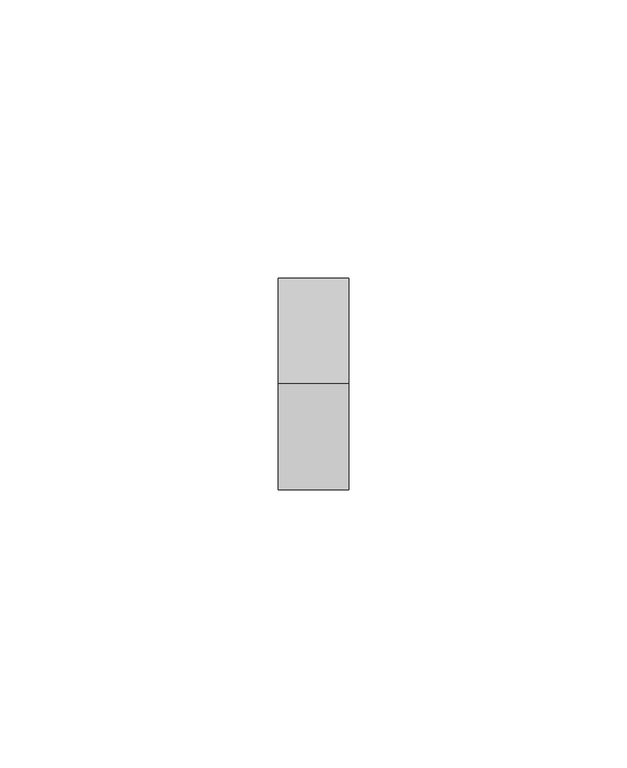
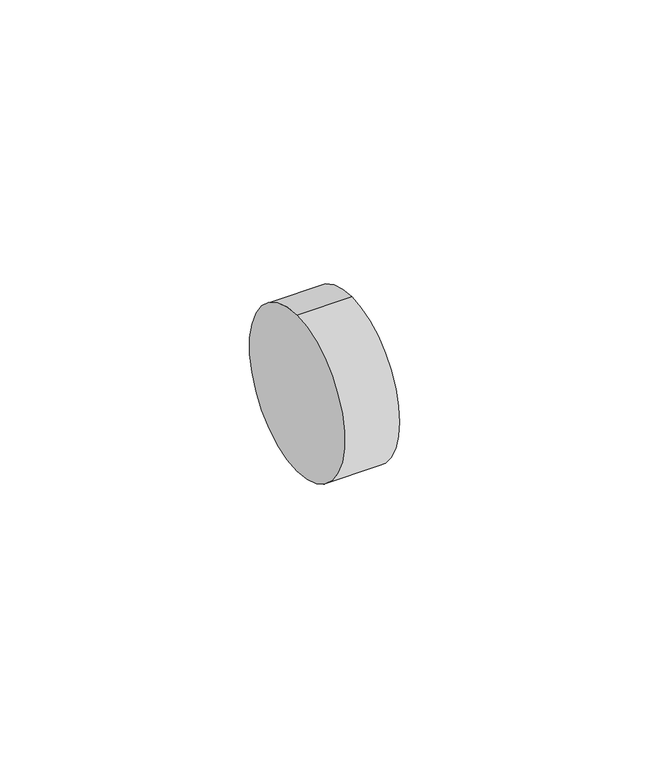
"""IFC4 building model written with IfcOpenShell, lengths in millimetres: proxy geometry, Bolt29:Bolt002:304741 : Bolt29:Bolt002:304741."""

from ifc_helpers import new_model, si_unit, point, frame, frame_2d, origin, place, context, project, spatial, circle_curve, trimmed, segment, composite_curve, outline, extrude, source, transform, mapped, element, save


def generic_models_d97a5a00(model_context):
    return source(origin(), model_context, "Body", "SweptSolid", [
        extrude(outline(composite_curve([segment(trimmed(circle_curve(frame_2d((2264.1630212, 39960.0063132)), 19.05), [point((2264.1630212, 39979.0563132))], [point((2264.1630212, 39940.9563132))], False, "CARTESIAN"), True, "CONTINUOUS"), segment(trimmed(circle_curve(frame_2d((2264.1630212, 39960.0063132)), 19.05), [point((2264.1630212, 39940.9563132))], [point((2264.1630212, 39979.0563132))], False, "CARTESIAN"), True, "CONTINUOUS")], self_intersect=False)), frame((15045.2731889, 0.0, 0.0), z_axis=(1.0, 0.0, 0.0), x_axis=(0.0, 1.0, 0.0)), (0.0, 0.0, 1.0), 12.7),
    ])


if __name__ == "__main__":
    model = new_model("IFC4")
    model_context = context("Model", 3, world=origin())
    ifc_project = project(units=[si_unit("LENGTHUNIT", "METRE", prefix="MILLI")], contexts=[model_context])
    site = spatial("IfcSite", under=ifc_project)
    building = spatial("IfcBuilding", under=site)
    placement = place(None, origin())
    generic_models_shape = generic_models_d97a5a00(model_context)
    element("IfcBuildingElementProxy", 1, Name="Bolt29:Bolt002:304741 : Bolt29:Bolt002:304741", ObjectType="Bolt29:Bolt002:304741 : Bolt29:Bolt002:304741", at=placement, inside=building, context=model_context, shape_type="MappedRepresentation", body=[
        mapped(generic_models_shape, transform((0.0, 0.0, 0.0), x_axis=(1.0, 0.0, 0.0), y_axis=(0.0, 1.0, 0.0), z_axis=(0.0, 0.0, 1.0))),
    ])
    save(model, "model.ifc")

# Revit data of these elements
# Type "Bolt29:Bolt002:304741 : Bolt29:Bolt002:304741"
#   NameOverride = "Bolt29:Bolt002:304741"
#   ObjectTypeOverride = "Bolt29:Bolt002"
#   Reference = "Bolt002"
#   Category = "Generic Models"
#   Tag = "304741"
# Element 1 (IfcBuildingElementProxy, "Bolt29:Bolt002:304741 : Bolt29:Bolt002:304741")
#   Materials on its faces: "TUBE STEEL STRINGER WELDED TO ANCHORED STEEL PLATE - SEE STRUCT DWGS"
# Materials
#   "TUBE STEEL STRINGER WELDED TO ANCHORED STEEL PLATE - SEE STRUCT DWGS": class "Unassigned", colour RGB 128 128 128, transparency 0, Cost = 0
